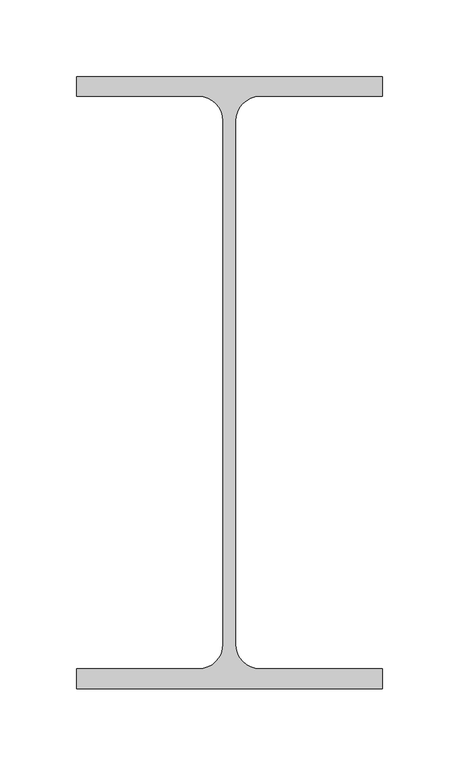
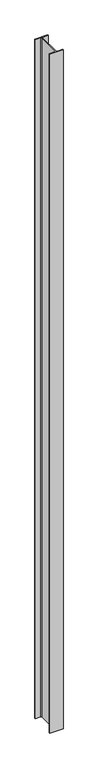
"""IFC4 building model written with IfcOpenShell, lengths in millimetres: column geometry, Steel Column_H_KSD3502 : H_SC_ASC_H-400x200x8x13."""

import ifcopenshell
import ifcopenshell.guid

model = None  # the IFC model being written
_history = None  # IfcOwnerHistory: only IFC2X3 demands one
_inside = {}  # id of a spatial element -> (the spatial element, [elements in it])
_under = {}  # id of a project, library or spatial element -> (it, [spatial elements below it])
_declared = {}  # id of a project -> (the project, [libraries it declares])
_typed = {}  # id of a type object -> (the type object, [elements of that type])
_made_of = {}  # id of a material, layer set ... -> (it, [elements and type objects made of it])


def new_model(schema):
    """Start an empty IFC model of exactly this schema.

    Asked for "IFC4X3", IfcOpenShell would pick the latest addendum, in which some entities
    have other attributes; the version numbers below select the first issue.
    IFC2X3 requires an IfcOwnerHistory on every rooted entity: one is made here for all.
    """
    global model, _history
    if schema == "IFC4X3":
        model = ifcopenshell.file(schema_version=(4, 3, 0, 0))
    else:
        model = ifcopenshell.file(schema=schema)
    _inside.clear()
    _under.clear()
    _declared.clear()
    _typed.clear()
    _made_of.clear()
    _history = None
    if model.schema == "IFC2X3":
        org = make("IfcOrganization", Name="unknown")
        user = make(
            "IfcPersonAndOrganization",
            ThePerson=make("IfcPerson", FamilyName="unknown"),
            TheOrganization=org,
        )
        app = make(
            "IfcApplication",
            ApplicationDeveloper=org,
            Version="unknown",
            ApplicationFullName="unknown",
            ApplicationIdentifier="unknown",
        )
        _history = make(
            "IfcOwnerHistory",
            OwningUser=user,
            OwningApplication=app,
            ChangeAction="ADDED",
            CreationDate=0,
        )
    return model


def make(cls, **values):
    """One entity of the class cls with the attributes given. An attribute that is None is left unset."""
    return model.create_entity(
        cls, **{name: value for name, value in values.items() if value is not None}
    )


def rooted(cls, **values):
    """An entity with a GlobalId (a new one), such as an element, a storey or a relation."""
    return make(cls, GlobalId=ifcopenshell.guid.new(), OwnerHistory=_history, **values)


def si_unit(unit_type, name, prefix=None):
    """IfcSIUnit, for example si_unit("LENGTHUNIT", "METRE", prefix="MILLI")."""
    return make("IfcSIUnit", UnitType=unit_type, Prefix=prefix, Name=name)


def assignment(units):
    """IfcUnitAssignment: the units of a project."""
    return None if units is None else make("IfcUnitAssignment", Units=units)


def point(xyz):
    """IfcCartesianPoint."""
    return None if xyz is None else make("IfcCartesianPoint", Coordinates=xyz)


def direction(xyz):
    """IfcDirection."""
    return None if xyz is None else make("IfcDirection", DirectionRatios=xyz)


def frame(location, z_axis=None, x_axis=None):
    """IfcAxis2Placement3D, a coordinate frame: its origin and axes. An axis left out is left unset."""
    return make(
        "IfcAxis2Placement3D",
        Location=point(location),
        Axis=direction(z_axis),
        RefDirection=direction(x_axis),
    )


def frame_2d(location, x_axis=None):
    """IfcAxis2Placement2D, a coordinate frame in the plane: its origin and x axis."""
    return make(
        "IfcAxis2Placement2D", Location=point(location), RefDirection=direction(x_axis)
    )


def origin():
    """The frame at (0, 0, 0) with its axes left unset."""
    return frame((0.0, 0.0, 0.0))


def place(relative_to, where):
    """IfcLocalPlacement: puts the frame where relative to a parent placement (None: the world)."""
    return make(
        "IfcLocalPlacement", PlacementRelTo=relative_to, RelativePlacement=where
    )


def context(
    kind, dimensions, precision=None, world=None, true_north=None, identifier=None
):
    """IfcGeometricRepresentationContext, for example the 3D "Model" context."""
    return make(
        "IfcGeometricRepresentationContext",
        ContextIdentifier=identifier,
        ContextType=kind,
        CoordinateSpaceDimension=dimensions,
        Precision=precision,
        WorldCoordinateSystem=world,
        TrueNorth=true_north,
    )


def project(units=None, contexts=None):
    """IfcProject with its units and contexts."""
    return rooted(
        "IfcProject",
        Name="project",
        RepresentationContexts=contexts,
        UnitsInContext=assignment(units),
    )


def spatial(cls, under=None, at=None, **own):
    """A site, building, storey or space (cls), placed at a placement, below another one or the project."""
    s = rooted(cls, ObjectPlacement=at, **own)
    if under is not None:
        _under.setdefault(under.id(), (under, []))[1].append(s)
    return s


def polyline(points):
    """IfcPolyline through the points."""
    return make("IfcPolyline", Points=[point(p) for p in points])


def circle_curve(where, radius):
    """IfcCircle in the frame where."""
    return make("IfcCircle", Position=where, Radius=radius)


def trimmed(basis, trim1, trim2, sense, master):
    """IfcTrimmedCurve: the piece of a basis curve between two trims."""
    return make(
        "IfcTrimmedCurve",
        BasisCurve=basis,
        Trim1=trim1,
        Trim2=trim2,
        SenseAgreement=sense,
        MasterRepresentation=master,
    )


def segment(curve, same_sense, transition):
    """IfcCompositeCurveSegment."""
    return make(
        "IfcCompositeCurveSegment",
        Transition=transition,
        SameSense=same_sense,
        ParentCurve=curve,
    )


def composite_curve(segments, self_intersect=None):
    """IfcCompositeCurve: segments joined end to end."""
    return make("IfcCompositeCurve", Segments=segments, SelfIntersect=self_intersect)


def outline(outer, holes=None, kind="AREA"):
    """IfcArbitraryClosedProfileDef: a profile drawn as a closed curve; with holes, ...WithVoids."""
    if holes is None:
        return make("IfcArbitraryClosedProfileDef", ProfileType=kind, OuterCurve=outer)
    return make(
        "IfcArbitraryProfileDefWithVoids",
        ProfileType=kind,
        OuterCurve=outer,
        InnerCurves=holes,
    )


def extrude(swept, where, along, depth):
    """IfcExtrudedAreaSolid: the profile swept, set in the frame where, extruded along a direction by depth."""
    return make(
        "IfcExtrudedAreaSolid",
        SweptArea=swept,
        Position=where,
        ExtrudedDirection=direction(along),
        Depth=depth,
    )


def shape(context_of_items, identifier, shape_type, items):
    """IfcShapeRepresentation: the items that make up one representation, for example the "Body"."""
    return make(
        "IfcShapeRepresentation",
        ContextOfItems=context_of_items,
        RepresentationIdentifier=identifier,
        RepresentationType=shape_type,
        Items=items,
    )


def source(mapping_origin, context_of_items, identifier, shape_type, items):
    """IfcRepresentationMap: a shape defined once, which mapped items show again and again."""
    return make(
        "IfcRepresentationMap",
        MappingOrigin=mapping_origin,
        MappedRepresentation=shape(context_of_items, identifier, shape_type, items),
    )


def transform(
    local_origin,
    x_axis=None,
    y_axis=None,
    z_axis=None,
    scale=None,
    scale2=None,
    scale3=None,
    uniform=True,
):
    """IfcCartesianTransformationOperator3D, or its non-uniform kind. x_axis, y_axis, z_axis: its Axis1, 2, 3."""
    if uniform:
        return make(
            "IfcCartesianTransformationOperator3D",
            Axis1=direction(x_axis),
            Axis2=direction(y_axis),
            LocalOrigin=point(local_origin),
            Scale=scale,
            Axis3=direction(z_axis),
        )
    return make(
        "IfcCartesianTransformationOperator3DnonUniform",
        Axis1=direction(x_axis),
        Axis2=direction(y_axis),
        LocalOrigin=point(local_origin),
        Scale=scale,
        Axis3=direction(z_axis),
        Scale2=scale2,
        Scale3=scale3,
    )


def mapped(mapping_source, mapping_target):
    """IfcMappedItem: shows the shape of a source again, moved by a transform."""
    return make(
        "IfcMappedItem", MappingSource=mapping_source, MappingTarget=mapping_target
    )


def made_of(thing, what):
    """Note that an element or type object is made of a material, layer set ...; save() writes the relation."""
    if what is not None:
        _made_of.setdefault(what.id(), (what, []))[1].append(thing)
    return thing


def element(
    cls,
    number,
    at=None,
    inside=None,
    cuts=None,
    type_object=None,
    material=None,
    context=None,
    identifier="Body",
    shape_type=None,
    held_by="IfcProductDefinitionShape",
    body=None,
    shapes=None,
    **own,
):
    """One element of the class cls, such as IfcWall. Its Tag is "e" and its number.

    at: its placement. inside: the storey or other place that contains it. cuts: it is an
    opening in that element (IfcRelVoidsElement). A single representation is given by context,
    identifier, shape_type and body (its items); several are given by shapes. held_by: the class
    of the entity that holds the representations. save() writes the other relations.
    """
    e = rooted(cls, Tag="e%d" % number, ObjectPlacement=at, **own)
    if body is not None:
        shapes = [shape(context, identifier, shape_type, body)]
    if shapes is not None:
        e.Representation = make(held_by, Representations=shapes)
    if inside is not None:
        _inside.setdefault(inside.id(), (inside, []))[1].append(e)
    if cuts is not None:
        rooted(
            "IfcRelVoidsElement", RelatingBuildingElement=cuts, RelatedOpeningElement=e
        )
    if type_object is not None:
        _typed.setdefault(type_object.id(), (type_object, []))[1].append(e)
    return made_of(e, material)


def aggregate(whole, parts):
    """IfcRelAggregates: a whole, such as a stair, and the parts it consists of."""
    return rooted("IfcRelAggregates", RelatingObject=whole, RelatedObjects=parts)


def save(model, path):
    """Write the relations noted so far, then the file.

    IfcRelAggregates (storeys below a building ...), IfcRelContainedInSpatialStructure (elements
    in a storey), IfcRelDefinesByType, IfcRelAssociatesMaterial and IfcRelDeclares: one each for
    every whole, place, type object, material and project.
    """
    for whole, parts in _under.values():
        aggregate(whole, parts)
    for where, things in _inside.values():
        rooted(
            "IfcRelContainedInSpatialStructure",
            RelatedElements=things,
            RelatingStructure=where,
        )
    for kind, things in _typed.values():
        rooted("IfcRelDefinesByType", RelatedObjects=things, RelatingType=kind)
    for what, things in _made_of.values():
        rooted("IfcRelAssociatesMaterial", RelatedObjects=things, RelatingMaterial=what)
    for by, libraries in _declared.values():
        rooted("IfcRelDeclares", RelatingContext=by, RelatedDefinitions=libraries)
    model.write(path)


def column_a45a25b2(model_context):
    return source(origin(), model_context, "Body", "SweptSolid", [
        extrude(outline(composite_curve([segment(polyline([(100.0, 200.0), (100.0, 187.0), (20.0, 187.0)]), True, "CONTINUOUS"), segment(trimmed(circle_curve(frame_2d((20.0, 171.0)), 16.0), [point((20.0, 187.0))], [point((4.0, 171.0))], True, "CARTESIAN"), True, "CONTINUOUS"), segment(polyline([(4.0, 171.0), (4.0, -171.0)]), True, "CONTINUOUS"), segment(trimmed(circle_curve(frame_2d((20.0, -171.0)), 16.0), [point((4.0, -171.0))], [point((20.0, -187.0))], True, "CARTESIAN"), True, "CONTINUOUS"), segment(polyline([(20.0, -187.0), (100.0, -187.0), (100.0, -200.0), (-100.0, -200.0), (-100.0, -187.0), (-20.0, -187.0)]), True, "CONTINUOUS"), segment(trimmed(circle_curve(frame_2d((-20.0, -171.0)), 16.0), [point((-20.0, -187.0))], [point((-4.0, -171.0))], True, "CARTESIAN"), True, "CONTINUOUS"), segment(polyline([(-4.0, -171.0), (-4.0, 171.0)]), True, "CONTINUOUS"), segment(trimmed(circle_curve(frame_2d((-20.0, 171.0)), 16.0), [point((-4.0, 171.0))], [point((-20.0, 187.0))], True, "CARTESIAN"), True, "CONTINUOUS"), segment(polyline([(-20.0, 187.0), (-100.0, 187.0), (-100.0, 200.0), (100.0, 200.0)]), True, "CONTINUOUS")], self_intersect=False)), frame((0.0, 0.0, 6649.9720055), z_axis=(0.0, 0.0, 1.0), x_axis=(1.0, 0.0, 0.0)), (0.0, 0.0, 1.0), 11000.0),
    ])


if __name__ == "__main__":
    model = new_model("IFC4")
    model_context = context("Model", 3, world=origin())
    ifc_project = project(units=[si_unit("LENGTHUNIT", "METRE", prefix="MILLI")], contexts=[model_context])
    site = spatial("IfcSite", under=ifc_project)
    building = spatial("IfcBuilding", under=site)
    placement = place(None, origin())
    column_shape = column_a45a25b2(model_context)
    element("IfcColumn", 1, ObjectType="Steel Column_H_KSD3502 : H_SC_ASC_H-400x200x8x13", at=placement, inside=building, context=model_context, shape_type="MappedRepresentation", body=[
        mapped(column_shape, transform((0.0, 0.0, 0.0), x_axis=(1.0, 0.0, 0.0), y_axis=(0.0, 1.0, 0.0), z_axis=(0.0, 0.0, 1.0))),
    ])
    save(model, "model.ifc")

# Revit data of these elements
# Type "Steel Column_H_KSD3502 : H_SC_ASC_H-400x200x8x13"
#   Width = 20.0 cm
#   Web Thickness = 0.8 cm
#   Web Fillet = 1.6 cm
#   Warping Constant = 648999.0 cm⁶
#   Torsional Moment of Inertia = 35.8981 cm⁴
#   Section Area = 84.12 cm²
#   Plastic Modulus weak axis = 268.0 cm³
#   Plastic Modulus strong axis = 1330.0 cm³
#   Perimeter = 1.27 m²/m
#   Nominal Weight = 66.00 kgf/m
#   Moment of Inertia weak axis = 1740.00 cm⁴
#   Moment of Inertia strong axis = 23700.00 cm⁴
#   Height = 40.0 cm
#   Flange Thickness = 1.3 cm
#   Elastic Modulus weak axis = 174.0 cm³
#   Elastic Modulus strong axis = 1190.0 cm³
#   Centroid Vertical = 20.0 cm
#   Centroid Horizontal = 10.0 cm
#   Bolt Spacing = 13.97 cm
#   Structural Material [instance default] = Steel, 45-345
#   Section Name Key = ""
#   Assembly Code = ""
# Element 1 (IfcColumn, "Steel Column_H_KSD3502 : H_SC_ASC_H-400x200x8x13")
#   Structural Material = none
# Materials
#   "Steel, 45-345": class "Metal", colour RGB 189 187 185, transparency 0, Description = "Steel 345 MPa", Cost = 0
